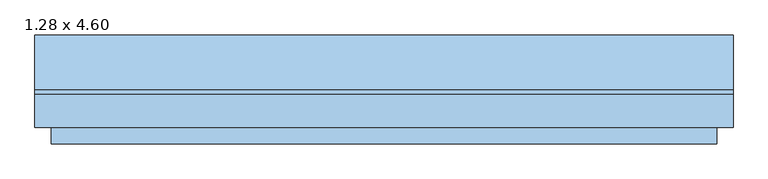
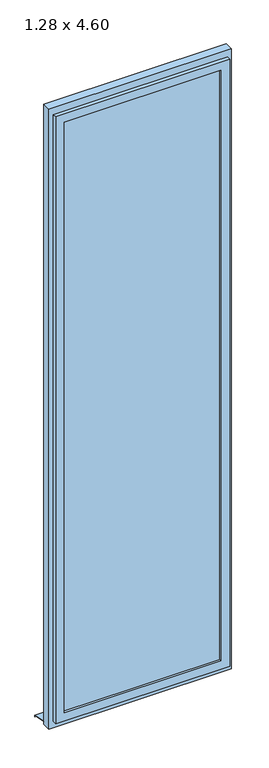
"""IFC4 building model written with IfcOpenShell, lengths in millimetres: window geometry, Fenstertür 1-flg : 1.28 x 4.60."""

from ifc_helpers import new_model, si_unit, frame, origin, place, context, project, spatial, polyline, outline, extrude, faceted_brep, source, transform, mapped, element, save


def window_1_28_x_4_60_0b6cddc5(model_context):
    return source(origin(), model_context, "Body", "SolidModel", [
        extrude(outline(polyline([(4600.0, 640.0), (4600.0, -640.0), (0.0, -640.0), (0.0, 640.0), (4600.0, 640.0)]), holes=[polyline([(4520.0, 580.0), (80.0, 580.0), (80.0, -580.0), (4520.0, -580.0), (4520.0, 580.0)])]), frame((0.0, -80.0, 0.0), z_axis=(0.0, 1.0, 0.0), x_axis=(0.0, 0.0, 1.0)), (0.0, 0.0, 1.0), 60.0),
        faceted_brep([(610.0, -80.0, 4550.0), (610.0, -110.0, 4550.0), (610.0, -110.0, 50.0), (610.0, -80.0, 50.0), (-610.0, -110.0, 4550.0), (-610.0, -110.0, 50.0), (550.0, -110.0, 110.0), (-550.0, -110.0, 110.0), (-550.0, -110.0, 4490.0), (550.0, -110.0, 4490.0), (-610.0, -80.0, 50.0), (-610.0, -80.0, 4550.0), (580.0, -80.0, 4520.0), (-580.0, -80.0, 4520.0), (-580.0, -80.0, 80.0), (580.0, -80.0, 80.0), (580.0, -50.0, 4520.0), (580.0, -50.0, 80.0), (-580.0, -50.0, 80.0), (-580.0, -50.0, 4520.0), (550.0, -50.0, 4490.0), (-550.0, -50.0, 4490.0), (-550.0, -50.0, 110.0), (550.0, -50.0, 110.0)], [[[0, 1, 2, 3]], [[1, 4, 5, 2], [6, 7, 8, 9]], [[3, 2, 5, 10]], [[3, 10, 11, 0], [12, 13, 14, 15]], [[16, 12, 15, 17]], [[17, 15, 14, 18]], [[17, 18, 19, 16], [20, 21, 22, 23]], [[9, 20, 23, 6]], [[6, 23, 22, 7]], [[10, 5, 4, 11]], [[18, 14, 13, 19]], [[7, 22, 21, 8]], [[11, 4, 1, 0]], [[19, 13, 12, 16]], [[8, 21, 20, 9]]]),
        extrude(outline(polyline([(-9.9778457, 20.0), (90.0, 0.0), (90.0, -10.0), (88.0, -10.0), (88.0, -1.6395366), (-10.1759277, 18.0), (-20.0, 18.0), (-20.0, 20.0), (-9.9778457, 20.0)])), frame((-640.0, 0.0, 0.0), z_axis=(1.0, 0.0, 0.0), x_axis=(0.0, 1.0, 0.0)), (0.0, 0.0, 1.0), 1280.0),
        extrude(outline(polyline([(550.0, -95.0), (-550.0, -95.0), (-550.0, -65.0), (550.0, -65.0), (550.0, -95.0)])), frame((0.0, 0.0, 110.0), z_axis=(0.0, 0.0, 1.0), x_axis=(1.0, 0.0, 0.0)), (0.0, 0.0, 1.0), 4380.0),
    ])


if __name__ == "__main__":
    model = new_model("IFC4")
    model_context = context("Model", 3, world=origin())
    ifc_project = project(units=[si_unit("LENGTHUNIT", "METRE", prefix="MILLI")], contexts=[model_context])
    site = spatial("IfcSite", under=ifc_project)
    building = spatial("IfcBuilding", under=site)
    placement = place(None, origin())
    window_1_28_x_4_60_shape = window_1_28_x_4_60_0b6cddc5(model_context)
    element("IfcWindow", 1, ObjectType="Fenstertür 1-flg : 1.28 x 4.60", at=placement, inside=building, context=model_context, shape_type="MappedRepresentation", body=[
        mapped(window_1_28_x_4_60_shape, transform((0.0, 0.0, 0.0), x_axis=(1.0, 0.0, 0.0), y_axis=(0.0, 1.0, 0.0), z_axis=(0.0, 0.0, 1.0))),
    ])
    save(model, "model.ifc")

# Revit data of these elements
# Project information
#   Projektausgabedatum = "Projekt Datum"
#   Projektstatus = "Projektstatus"
#   Kundenname = "Bauherr"
#   Projektadresse = "Projektadresse"
#   Projektname = "Projektname"
#   Projektnummer = "Projektnummer"
#   Verfasser Firma 1 = "Firma 1"
#   Verfasser Firma 2 = "Firma 2"
#   Verfasser PLZ Ort = "PLZ Ort"
#   Verfasser Strasse = "Strasse"
#   Verfasser Telefon = "Telefon"
#   Verfasser Telefax = "Telefax"
#   Verfasser eMail = "E-Mail"
# Type "Fenstertür 1-flg : 1.28 x 4.60"
#   Type Mark = "58"
#   Operation = "SinglePanel"
#   Construction Type Id = "SGL"
#   Keynote = "16.05.01"
#   Analytic Construction = "Große Fenster mit Einfachverglasung"
#   Visual Light Transmittance = 0.9
#   Solar Heat Gain Coefficient = 0.86
#   Rough Width = 1.280 m
#   Rough Height = 4.600 m
#   Heat Transfer Coefficient (U) = 5.5617 W/(m²·K)
#   Rahmentiefe = 0.060 m
#   Rahmenhöhe unten = 0.080 m
#   Höhe oberer  Rahmen = 0.080 m
#   Rahmenbreite = 0.060 m
#   Height = 4.600 m
#   Tiefe Flügel = 0.060 m
#   Flügelbreite = 0.060 m
#   Einbautiefe (von außen) [instance default] = 0.080 m
#   Width = 1.280 m
#   Sichtbarkeit Sturzlinien [instance default] = yes
#   Öffnungsrichtung oben [instance default] = yes
#   Öffnungsrichtung in Draufsicht anzeigen [instance default] = yes
#   Drehflügel 1 [instance default] = yes
#   Bild [instance default] = none
#   Glas [instance default] = none
#   Fensterflügel [instance default] = none
#   Äußere Fensterbank [instance default] = none
#   Wall Closure = (empty or 0)
# Element 1 (IfcWindow, "Fenstertür 1-flg : 1.28 x 4.60")
#   Materials on its faces: "Kunststoff - Weiß", "Glas"
# Materials
#   "Kunststoff - Weiß": class "Kunststoff", colour RGB 249 249 249, transparency 0, Cost = 0
#   "Glas": class "Glas", colour RGB 0 0 255, transparency 0.75, Comments = "Render-Darstellung nicht aktualisiert ", Cost = 0
